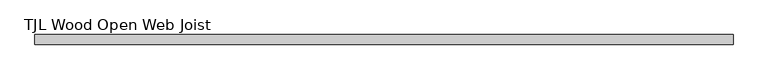
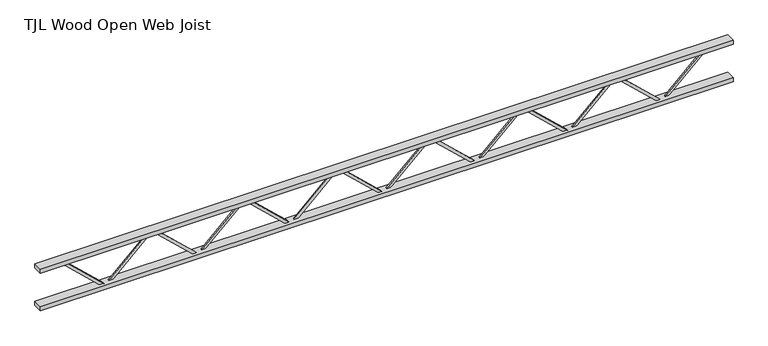
"""IFC4 building model written with IfcOpenShell, lengths in millimetres: beam geometry, TJL Wood Open Web Joist."""

from ifc_helpers import new_model, si_unit, frame, origin, place, context, project, spatial, polyline, outline, extrude, source, transform, mapped, element, save


def tjl_wood_open_web_joist_102efcec(model_context):
    return source(origin(), model_context, "Body", "SweptSolid", [
        extrude(outline(polyline([(171.45, 2152.7633929), (196.85, 2152.7633929), (196.85, 2135.0374708), (-171.45, 1742.5847923), (-171.45, 1696.8107143), (-196.85, 1696.8107143), (-196.85, 1752.6366363), (171.45, 2145.0893149), (171.45, 2152.7633929)])), frame((0.0, 0.0, 0.0), z_axis=(0.0, 1.0, 0.0), x_axis=(0.0, 0.0, 1.0)), (0.0, 0.0, 1.0), 12.7),
        extrude(outline(polyline([(196.85, 1291.6580357), (171.45, 1291.6580357), (171.45, 1299.3321137), (-196.85, 1691.7847923), (-196.85, 1747.6107143), (-171.45, 1747.6107143), (-171.45, 1701.8366363), (196.85, 1309.3839577), (196.85, 1291.6580357)])), frame((0.0, -12.7, 0.0), z_axis=(0.0, 1.0, 0.0), x_axis=(0.0, 0.0, 1.0)), (0.0, 0.0, 1.0), 12.7),
        extrude(outline(polyline([(171.45, 1291.6580357), (196.85, 1291.6580357), (196.85, 1273.9321137), (-171.45, 881.4794351), (-171.45, 835.7053571), (-196.85, 835.7053571), (-196.85, 891.5312792), (171.45, 1283.9839577), (171.45, 1291.6580357)])), frame((0.0, 0.0, 0.0), z_axis=(0.0, 1.0, 0.0), x_axis=(0.0, 0.0, 1.0)), (0.0, 0.0, 1.0), 12.7),
        extrude(outline(polyline([(196.85, 430.5526786), (171.45, 430.5526786), (171.45, 438.2267565), (-196.85, 830.6794351), (-196.85, 886.5053571), (-171.45, 886.5053571), (-171.45, 840.7312792), (196.85, 448.2786006), (196.85, 430.5526786)])), frame((0.0, -12.7, 0.0), z_axis=(0.0, 1.0, 0.0), x_axis=(0.0, 0.0, 1.0)), (0.0, 0.0, 1.0), 12.7),
        extrude(outline(polyline([(171.45, 430.5526786), (196.85, 430.5526786), (196.85, 412.8267565), (-171.45, 20.374078), (-171.45, -25.4), (-196.85, -25.4), (-196.85, 30.425922), (171.45, 422.8786006), (171.45, 430.5526786)])), frame((0.0, 0.0, 0.0), z_axis=(0.0, 1.0, 0.0), x_axis=(0.0, 0.0, 1.0)), (0.0, 0.0, 1.0), 12.7),
        extrude(outline(polyline([(196.85, -430.5526786), (171.45, -430.5526786), (171.45, -422.8786006), (-196.85, -30.425922), (-196.85, 25.4), (-171.45, 25.4), (-171.45, -20.374078), (196.85, -412.8267565), (196.85, -430.5526786)])), frame((0.0, -12.7, 0.0), z_axis=(0.0, 1.0, 0.0), x_axis=(0.0, 0.0, 1.0)), (0.0, 0.0, 1.0), 12.7),
        extrude(outline(polyline([(171.45, -430.5526786), (196.85, -430.5526786), (196.85, -448.2786006), (-171.45, -840.7312792), (-171.45, -886.5053571), (-196.85, -886.5053571), (-196.85, -830.6794351), (171.45, -438.2267565), (171.45, -430.5526786)])), frame((0.0, 0.0, 0.0), z_axis=(0.0, 1.0, 0.0), x_axis=(0.0, 0.0, 1.0)), (0.0, 0.0, 1.0), 12.7),
        extrude(outline(polyline([(196.85, -1291.6580357), (171.45, -1291.6580357), (171.45, -1283.9839577), (-196.85, -891.5312792), (-196.85, -835.7053571), (-171.45, -835.7053571), (-171.45, -881.4794351), (196.85, -1273.9321137), (196.85, -1291.6580357)])), frame((0.0, -12.7, 0.0), z_axis=(0.0, 1.0, 0.0), x_axis=(0.0, 0.0, 1.0)), (0.0, 0.0, 1.0), 12.7),
        extrude(outline(polyline([(171.45, -1291.6580357), (196.85, -1291.6580357), (196.85, -1309.3839577), (-171.45, -1701.8366363), (-171.45, -1747.6107143), (-196.85, -1747.6107143), (-196.85, -1691.7847923), (171.45, -1299.3321137), (171.45, -1291.6580357)])), frame((0.0, 0.0, 0.0), z_axis=(0.0, 1.0, 0.0), x_axis=(0.0, 0.0, 1.0)), (0.0, 0.0, 1.0), 12.7),
        extrude(outline(polyline([(196.85, -2152.7633929), (171.45, -2152.7633929), (171.45, -2145.0893149), (-196.85, -1752.6366363), (-196.85, -1696.8107143), (-171.45, -1696.8107143), (-171.45, -1742.5847923), (196.85, -2135.0374708), (196.85, -2152.7633929)])), frame((0.0, -12.7, 0.0), z_axis=(0.0, 1.0, 0.0), x_axis=(0.0, 0.0, 1.0)), (0.0, 0.0, 1.0), 12.7),
        extrude(outline(polyline([(171.45, 3013.86875), (196.85, 3013.86875), (196.85, 2996.142828), (-171.45, 2603.6901494), (-171.45, 2557.9160714), (-196.85, 2557.9160714), (-196.85, 2613.7419935), (171.45, 3006.194672), (171.45, 3013.86875)])), frame((0.0, 0.0, 0.0), z_axis=(0.0, 1.0, 0.0), x_axis=(0.0, 0.0, 1.0)), (0.0, 0.0, 1.0), 12.7),
        extrude(outline(polyline([(196.85, 2152.7633929), (171.45, 2152.7633929), (171.45, 2160.4374708), (-196.85, 2552.8901494), (-196.85, 2608.7160714), (-171.45, 2608.7160714), (-171.45, 2562.9419935), (196.85, 2170.4893149), (196.85, 2152.7633929)])), frame((0.0, -12.7, 0.0), z_axis=(0.0, 1.0, 0.0), x_axis=(0.0, 0.0, 1.0)), (0.0, 0.0, 1.0), 12.7),
        extrude(outline(polyline([(171.45, -2152.7633929), (196.85, -2152.7633929), (196.85, -2170.4893149), (-171.45, -2562.9419935), (-171.45, -2608.7160714), (-196.85, -2608.7160714), (-196.85, -2552.8901494), (171.45, -2160.4374708), (171.45, -2152.7633929)])), frame((0.0, 0.0, 0.0), z_axis=(0.0, 1.0, 0.0), x_axis=(0.0, 0.0, 1.0)), (0.0, 0.0, 1.0), 12.7),
        extrude(outline(polyline([(196.85, -3013.86875), (171.45, -3013.86875), (171.45, -3006.194672), (-196.85, -2613.7419935), (-196.85, -2557.9160714), (-171.45, -2557.9160714), (-171.45, -2603.6901494), (196.85, -2996.142828), (196.85, -3013.86875)])), frame((0.0, -12.7, 0.0), z_axis=(0.0, 1.0, 0.0), x_axis=(0.0, 0.0, 1.0)), (0.0, 0.0, 1.0), 12.7),
        extrude(outline(polyline([(3217.06875, 44.45), (3217.06875, -44.45), (-3217.06875, -44.45), (-3217.06875, 44.45), (3217.06875, 44.45)])), frame((0.0, 0.0, 165.1), z_axis=(0.0, 0.0, 1.0), x_axis=(1.0, 0.0, 0.0)), (0.0, 0.0, 1.0), 38.1),
        extrude(outline(polyline([(3217.06875, 44.45), (3217.06875, -44.45), (-3217.06875, -44.45), (-3217.06875, 44.45), (3217.06875, 44.45)])), frame((0.0, 0.0, -203.2), z_axis=(0.0, 0.0, 1.0), x_axis=(1.0, 0.0, 0.0)), (0.0, 0.0, 1.0), 38.1),
    ])


if __name__ == "__main__":
    model = new_model("IFC4")
    model_context = context("Model", 3, world=origin())
    ifc_project = project(units=[si_unit("LENGTHUNIT", "METRE", prefix="MILLI")], contexts=[model_context])
    site = spatial("IfcSite", under=ifc_project)
    building = spatial("IfcBuilding", under=site)
    placement = place(None, origin())
    tjl_wood_open_web_joist_shape = tjl_wood_open_web_joist_102efcec(model_context)
    element("IfcBeam", 1, ObjectType="TJL Wood Open Web Joist : 16\" PREENGINEERED FLOOR TRUSS", at=placement, inside=building, context=model_context, shape_type="MappedRepresentation", body=[
        mapped(tjl_wood_open_web_joist_shape, transform((0.0, 0.0, 0.0), x_axis=(1.0, 0.0, 0.0), y_axis=(0.0, 1.0, 0.0), z_axis=(0.0, 0.0, 1.0))),
    ])
    save(model, "model.ifc")

# Revit data of these elements
# Type "TJL Wood Open Web Joist : 16\" PREENGINEERED FLOOR TRUSS"
#   Web Thickness = 0' - 1"
#   Web Leg = 0' - 1"
#   Start Offset [instance default] = 0' - 0"
#   Top Chord Start Extension [instance default] = 0' - 0"
#   PanelArrayLength [instance default] = 22' - 8"
#   Depth = 1' - 4"
#   PanelWidth [instance default] = 2' - 6.22222"
#   Offset Length 2 [instance default] = 0' - 8"
#   Offset Length 1 [instance default] = 0' - 8"
#   End Panel [instance default] = 0' - 8"
#   End Offset [instance default] = 0' - 0"
#   Top Chord End Extension [instance default] = 0' - 0"
#   Chord Width = 0' - 3 1/2"
#   Chord Depth = 0' - 1 1/2"
#   Bottom Chord Start Extension [instance default] = 0' - 0"
#   Bottom Chord End Extension [instance default] = 0' - 0"
#   Length [instance default] = 24' - 0"
#   PanelArrayNum [instance default] = 9
#   Web Rendering Material = none
#   Structural Material = none
#   Assembly Code = ""
# Element 1 (IfcBeam, "TJL Wood Open Web Joist : 16\" PREENGINEERED FLOOR TRUSS")
#   PanelArrayLength = 19' - 9 5/16"
#   PanelWidth = 2' - 9.90179"
#   PanelArrayNum = 7
